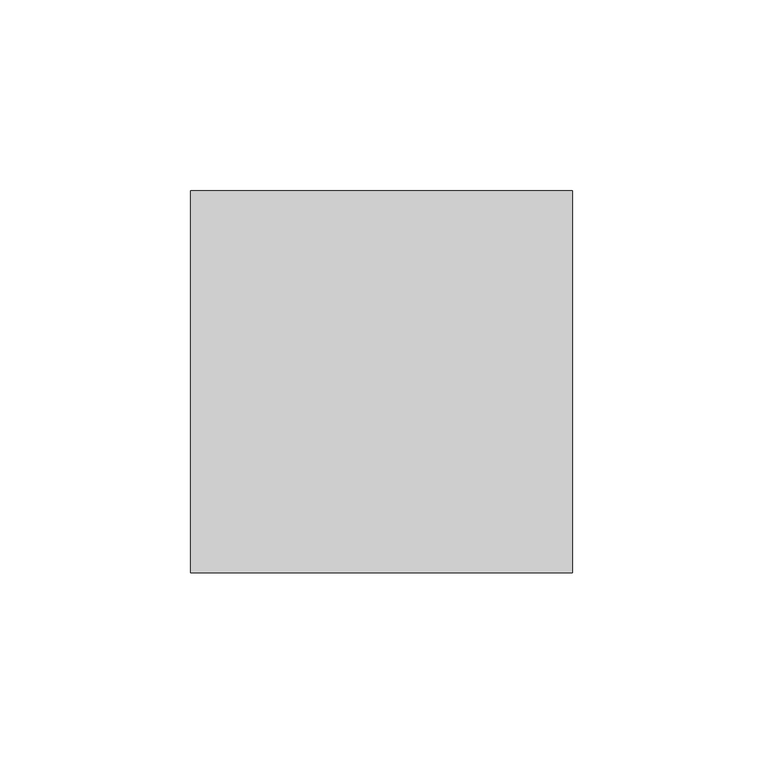
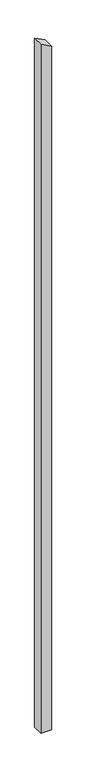
"""IFC4 building model written with IfcOpenShell, lengths in millimetres: column geometry, Holzstütze 159156 : Holzstütze 159156."""

from ifc_helpers import new_model, si_unit, frame, origin, place, context, project, spatial, polyline, outline, extrude, source, transform, mapped, element, save


def column_28b62d45(model_context):
    return source(origin(), model_context, "Body", "SweptSolid", [
        extrude(outline(polyline([(-500.0, 174197.7593015), (-500.0, 174297.7593015), (6345.7118258, 174297.7593015), (6396.6643707, 174197.7593015), (-500.0, 174197.7593015)])), frame((0.0, 33138.3551606, 0.0), z_axis=(0.0, 1.0, 0.0), x_axis=(0.0, 0.0, 1.0)), (0.0, 0.0, 1.0), 100.0),
    ])


if __name__ == "__main__":
    model = new_model("IFC4")
    model_context = context("Model", 3, world=origin())
    ifc_project = project(units=[si_unit("LENGTHUNIT", "METRE", prefix="MILLI")], contexts=[model_context])
    site = spatial("IfcSite", under=ifc_project)
    building = spatial("IfcBuilding", under=site)
    placement = place(None, origin())
    column_shape = column_28b62d45(model_context)
    element("IfcColumn", 1, ObjectType="Holzstütze 159156 : Holzstütze 159156", at=placement, inside=building, context=model_context, shape_type="MappedRepresentation", body=[
        mapped(column_shape, transform((0.0, 0.0, 0.0), x_axis=(1.0, 0.0, 0.0), y_axis=(0.0, 1.0, 0.0), z_axis=(0.0, 0.0, 1.0))),
    ])
    save(model, "model.ifc")

# Revit data of these elements
# Type "Holzstütze 159156 : Holzstütze 159156"
#   Abrechnungsart = "m"
#   Allright_Bauteil_ID = "0152St 0000143360"
#   Bezeichnung = "Holzstütze"
#   Codetext = "ST-HOLZ\\"
#   Gewerk = "Zimmer- und Holzbauarbeiten"
#   Material = "Holz"
#   Objektname = "Stütze"
#   NameOverride = "Holzstütze"
#   Reference = "Holzstütze"
#   Status = "NEW"
#   ThermalTransmittance = 0.0000 BTU/(h·ft²·°F)
#   Roll = 0.00°
#   Slope = 0.00°
#   2D Interaktion = yes
#   IsExternal = yes
#   LoadBearing = yes
# Element 1 (IfcColumn, "Holzstütze 159156 : Holzstütze 159156")
#   Materials on its faces: "holzschalung"
# Materials
#   "holzschalung": class "Unassigned", colour RGB 128 128 128, transparency 0
